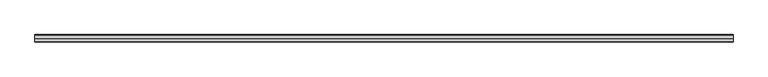
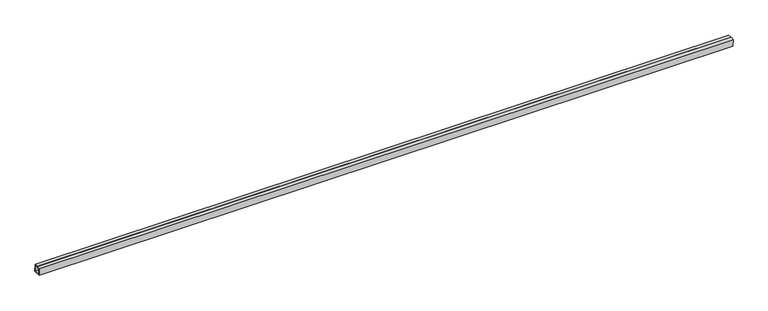
"""IFC4 building model written with IfcOpenShell, lengths in millimetres: proxy geometry, Inner panel:Inner panel:1:Inner panel:1 : Inner panel:Inner panel:300324:2:Inner panel:1:Inner panel:1 : Inner panel:Inner panel:300324:2 : Inner panel:Inner panel:1:Inner panel:1 : Inner panel:Inner panel:300324:300043:38 : Inner panel:Inner panel:1:Inner panel:1 : Inner panel:Inner panel:300324:2:Inner panel:1:Inner panel:1 : Inner panel:Inner panel:300324:2 : Inner panel:Inner panel:1:Inner panel:1 : Inner panel:Inner panel:300324:300043:308120."""

from ifc_helpers import new_model, si_unit, frame, origin, place, context, project, spatial, polyline, outline, extrude, source, transform, mapped, element, save


def generic_models_19f3e373(model_context):
    return source(origin(), model_context, "Body", "SweptSolid", [
        extrude(outline(polyline([(-581211.0091179, 3857.8017792), (-581192.7686948, 3858.5617968), (-581191.182571, 3820.4948267), (-581229.2495411, 3818.908703), (-581230.8356649, 3856.9756731), (-581212.5952417, 3857.7356907), (-581212.496109, 3855.3565051), (-581228.3573465, 3854.6956202), (-581226.9694882, 3821.3870213), (-581193.6608894, 3822.7748796), (-581195.0487477, 3856.0834785), (-581210.9099852, 3855.4225936), (-581211.0091179, 3857.8017792)])), frame((612749.9867239, 0.0, 0.0), z_axis=(1.0, 0.0, 0.0), x_axis=(0.0, 1.0, 0.0)), (0.0, 0.0, 1.0), 3657.6),
    ])


if __name__ == "__main__":
    model = new_model("IFC4")
    model_context = context("Model", 3, world=origin())
    ifc_project = project(units=[si_unit("LENGTHUNIT", "METRE", prefix="MILLI")], contexts=[model_context])
    site = spatial("IfcSite", under=ifc_project)
    building = spatial("IfcBuilding", under=site)
    placement = place(None, origin())
    generic_models_shape = generic_models_19f3e373(model_context)
    element("IfcBuildingElementProxy", 1, Name="Inner panel:Inner panel:1:Inner panel:1 : Inner panel:Inner panel:300324:2:Inner panel:1:Inner panel:1 : Inner panel:Inner panel:300324:2 : Inner panel:Inner panel:1:Inner panel:1 : Inner panel:Inner panel:300324:300043:38 : Inner panel:Inner panel:1:Inner panel:1 : Inner panel:Inner panel:300324:2:Inner panel:1:Inner panel:1 : Inner panel:Inner panel:300324:2 : Inner panel:Inner panel:1:Inner panel:1 : Inner panel:Inner panel:300324:300043:308120", ObjectType="Inner panel:Inner panel:1:Inner panel:1 : Inner panel:Inner panel:300324:2:Inner panel:1:Inner panel:1 : Inner panel:Inner panel:300324:2 : Inner panel:Inner panel:1:Inner panel:1 : Inner panel:Inner panel:300324:300043:38 : Inner panel:Inner panel:1:Inner panel:1 : Inner panel:Inner panel:300324:2:Inner panel:1:Inner panel:1 : Inner panel:Inner panel:300324:2 : Inner panel:Inner panel:1:Inner panel:1 : Inner panel:Inner panel:300324:300043:308120", at=placement, inside=building, context=model_context, shape_type="MappedRepresentation", body=[
        mapped(generic_models_shape, transform((0.0, 0.0, 0.0), x_axis=(1.0, 0.0, 0.0), y_axis=(0.0, 1.0, 0.0), z_axis=(0.0, 0.0, 1.0))),
    ])
    save(model, "model.ifc")

# Revit data of these elements
# Type "Inner panel:Inner panel:1:Inner panel:1 : Inner panel:Inner panel:300324:2:Inner panel:1:Inner panel:1 : Inner panel:Inner panel:300324:2 : Inner panel:Inner panel:1:Inner panel:1 : Inner panel:Inner panel:300324:300043:38 : Inner panel:Inner panel:1:Inner panel:1 : Inner panel:Inner panel:300324:2:Inner panel:1:Inner panel:1 : Inner panel:Inner panel:300324:2 : Inner panel:Inner panel:1:Inner panel:1 : Inner panel:Inner panel:300324:300043:308120"
#   NameOverride = "Inner panel:Inner panel:1:Inner panel:1 : Inner panel:Inner panel:300324:2:Inner panel:1:Inner panel:1 : Inner panel:Inner panel:300324:2 : Inner panel:Inner panel:1:Inner panel:1 : Inner panel:Inner panel:300324:300043:308120"
#   ObjectTypeOverride = "Inner panel:1:Inner panel:1 : Inner panel:Inner panel:300324:2 : Inner panel:Inner panel:1:Inner panel:1 : Inner panel:Inner panel:300324:300043"
#   Reference = "Inner panel"
#   Tag = "308120"
# Element 1 (IfcBuildingElementProxy, "Inner panel:Inner panel:1:Inner panel:1 : Inner panel:Inner panel:300324:2:Inner panel:1:Inner panel:1 : Inner panel:Inner panel:300324:2 : Inner panel:Inner panel:1:Inner panel:1 : Inner panel:Inner panel:300324:300043:38 : Inner panel:Inner panel:1:Inner panel:1 : Inner panel:Inner panel:300324:2:Inner panel:1:Inner panel:1 : Inner panel:Inner panel:300324:2 : Inner panel:Inner panel:1:Inner panel:1 : Inner panel:Inner panel:300324:300043:308120")
#   Materials on its faces: "1 1/2\" X 1 1/2\" SPLIT-SEAM SQUARE TUBING (~24\" CANTILEVER FROM C.L. OF GLULAM)"
# Materials
#   "1 1/2\" X 1 1/2\" SPLIT-SEAM SQUARE TUBING (~24\" CANTILEVER FROM C.L. OF GLULAM)": class "Unassigned", colour RGB 202 201 200, transparency 0, Cost = 0
